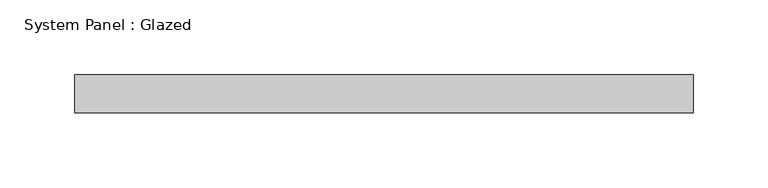
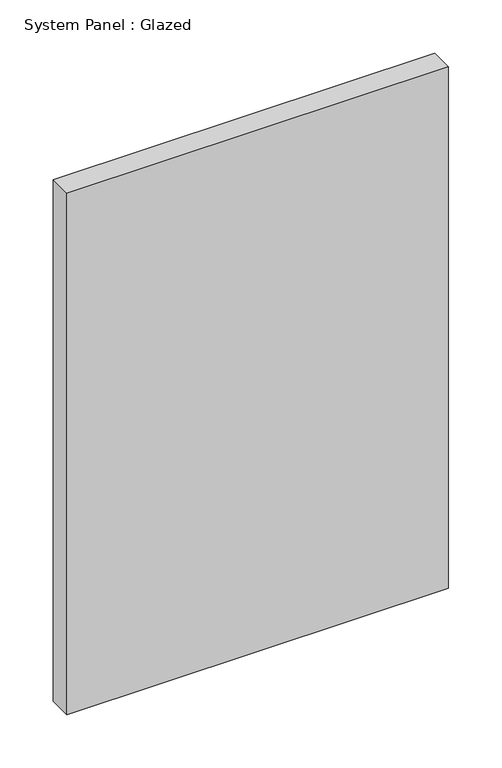
"""IFC4 building model written with IfcOpenShell, lengths in millimetres: plate geometry, System Panel : Glazed."""

from ifc_helpers import new_model, si_unit, origin, origin_with_axes, place, context, project, spatial, polyline, outline, extrude, source, transform, mapped, element, save


def system_panel_glazed_17866f5f(model_context):
    return source(origin(), model_context, "Body", "SweptSolid", [
        extrude(outline(polyline([(206.3749998, 19.05), (-206.3749998, 19.05), (-206.3749998, 44.45), (206.3749998, 44.45), (206.3749998, 19.05)])), origin_with_axes(), (0.0, 0.0, 1.0), 596.9),
    ])


if __name__ == "__main__":
    model = new_model("IFC4")
    model_context = context("Model", 3, world=origin())
    ifc_project = project(units=[si_unit("LENGTHUNIT", "METRE", prefix="MILLI")], contexts=[model_context])
    site = spatial("IfcSite", under=ifc_project)
    building = spatial("IfcBuilding", under=site)
    placement = place(None, origin())
    system_panel_glazed_shape = system_panel_glazed_17866f5f(model_context)
    element("IfcPlate", 1, ObjectType="System Panel : Glazed", at=placement, inside=building, context=model_context, shape_type="MappedRepresentation", body=[
        mapped(system_panel_glazed_shape, transform((0.0, 0.0, 0.0), x_axis=(1.0, 0.0, 0.0), y_axis=(0.0, 1.0, 0.0), z_axis=(0.0, 0.0, 1.0))),
    ])
    save(model, "model.ifc")

# Revit data of these elements
# Element 1 (IfcPlate, "System Panel : Glazed")
#   Materials on its faces: "Glass"
# Materials
#   "Glass": class "Glass", colour RGB 0 128 192, transparency 0.75
